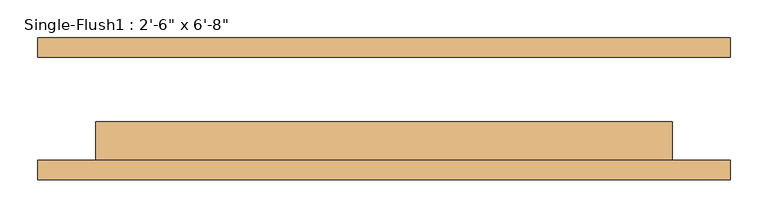
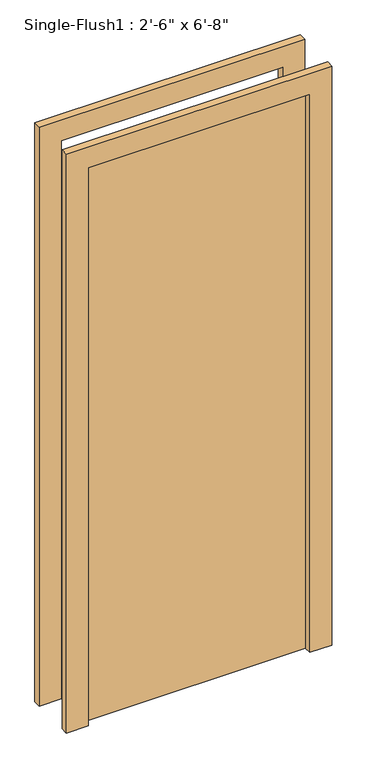
"""IFC4 building model written with IfcOpenShell, lengths in millimetres: door geometry."""

import ifcopenshell
import ifcopenshell.guid

model = None  # the IFC model being written
_history = None  # IfcOwnerHistory: only IFC2X3 demands one
_inside = {}  # id of a spatial element -> (the spatial element, [elements in it])
_under = {}  # id of a project, library or spatial element -> (it, [spatial elements below it])
_declared = {}  # id of a project -> (the project, [libraries it declares])
_typed = {}  # id of a type object -> (the type object, [elements of that type])
_made_of = {}  # id of a material, layer set ... -> (it, [elements and type objects made of it])


def new_model(schema):
    """Start an empty IFC model of exactly this schema.

    Asked for "IFC4X3", IfcOpenShell would pick the latest addendum, in which some entities
    have other attributes; the version numbers below select the first issue.
    IFC2X3 requires an IfcOwnerHistory on every rooted entity: one is made here for all.
    """
    global model, _history
    if schema == "IFC4X3":
        model = ifcopenshell.file(schema_version=(4, 3, 0, 0))
    else:
        model = ifcopenshell.file(schema=schema)
    _inside.clear()
    _under.clear()
    _declared.clear()
    _typed.clear()
    _made_of.clear()
    _history = None
    if model.schema == "IFC2X3":
        org = make("IfcOrganization", Name="unknown")
        user = make(
            "IfcPersonAndOrganization",
            ThePerson=make("IfcPerson", FamilyName="unknown"),
            TheOrganization=org,
        )
        app = make(
            "IfcApplication",
            ApplicationDeveloper=org,
            Version="unknown",
            ApplicationFullName="unknown",
            ApplicationIdentifier="unknown",
        )
        _history = make(
            "IfcOwnerHistory",
            OwningUser=user,
            OwningApplication=app,
            ChangeAction="ADDED",
            CreationDate=0,
        )
    return model


def make(cls, **values):
    """One entity of the class cls with the attributes given. An attribute that is None is left unset."""
    return model.create_entity(
        cls, **{name: value for name, value in values.items() if value is not None}
    )


def rooted(cls, **values):
    """An entity with a GlobalId (a new one), such as an element, a storey or a relation."""
    return make(cls, GlobalId=ifcopenshell.guid.new(), OwnerHistory=_history, **values)


def si_unit(unit_type, name, prefix=None):
    """IfcSIUnit, for example si_unit("LENGTHUNIT", "METRE", prefix="MILLI")."""
    return make("IfcSIUnit", UnitType=unit_type, Prefix=prefix, Name=name)


def assignment(units):
    """IfcUnitAssignment: the units of a project."""
    return None if units is None else make("IfcUnitAssignment", Units=units)


def point(xyz):
    """IfcCartesianPoint."""
    return None if xyz is None else make("IfcCartesianPoint", Coordinates=xyz)


def direction(xyz):
    """IfcDirection."""
    return None if xyz is None else make("IfcDirection", DirectionRatios=xyz)


def frame(location, z_axis=None, x_axis=None):
    """IfcAxis2Placement3D, a coordinate frame: its origin and axes. An axis left out is left unset."""
    return make(
        "IfcAxis2Placement3D",
        Location=point(location),
        Axis=direction(z_axis),
        RefDirection=direction(x_axis),
    )


def origin():
    """The frame at (0, 0, 0) with its axes left unset."""
    return frame((0.0, 0.0, 0.0))


def origin_with_axes():
    """The frame at (0, 0, 0) with the z axis (0, 0, 1) and the x axis (1, 0, 0) written out."""
    return frame((0.0, 0.0, 0.0), z_axis=(0.0, 0.0, 1.0), x_axis=(1.0, 0.0, 0.0))


def place(relative_to, where):
    """IfcLocalPlacement: puts the frame where relative to a parent placement (None: the world)."""
    return make(
        "IfcLocalPlacement", PlacementRelTo=relative_to, RelativePlacement=where
    )


def context(
    kind, dimensions, precision=None, world=None, true_north=None, identifier=None
):
    """IfcGeometricRepresentationContext, for example the 3D "Model" context."""
    return make(
        "IfcGeometricRepresentationContext",
        ContextIdentifier=identifier,
        ContextType=kind,
        CoordinateSpaceDimension=dimensions,
        Precision=precision,
        WorldCoordinateSystem=world,
        TrueNorth=true_north,
    )


def project(units=None, contexts=None):
    """IfcProject with its units and contexts."""
    return rooted(
        "IfcProject",
        Name="project",
        RepresentationContexts=contexts,
        UnitsInContext=assignment(units),
    )


def spatial(cls, under=None, at=None, **own):
    """A site, building, storey or space (cls), placed at a placement, below another one or the project."""
    s = rooted(cls, ObjectPlacement=at, **own)
    if under is not None:
        _under.setdefault(under.id(), (under, []))[1].append(s)
    return s


def polyline(points):
    """IfcPolyline through the points."""
    return make("IfcPolyline", Points=[point(p) for p in points])


def outline(outer, holes=None, kind="AREA"):
    """IfcArbitraryClosedProfileDef: a profile drawn as a closed curve; with holes, ...WithVoids."""
    if holes is None:
        return make("IfcArbitraryClosedProfileDef", ProfileType=kind, OuterCurve=outer)
    return make(
        "IfcArbitraryProfileDefWithVoids",
        ProfileType=kind,
        OuterCurve=outer,
        InnerCurves=holes,
    )


def extrude(swept, where, along, depth):
    """IfcExtrudedAreaSolid: the profile swept, set in the frame where, extruded along a direction by depth."""
    return make(
        "IfcExtrudedAreaSolid",
        SweptArea=swept,
        Position=where,
        ExtrudedDirection=direction(along),
        Depth=depth,
    )


def shape(context_of_items, identifier, shape_type, items):
    """IfcShapeRepresentation: the items that make up one representation, for example the "Body"."""
    return make(
        "IfcShapeRepresentation",
        ContextOfItems=context_of_items,
        RepresentationIdentifier=identifier,
        RepresentationType=shape_type,
        Items=items,
    )


def source(mapping_origin, context_of_items, identifier, shape_type, items):
    """IfcRepresentationMap: a shape defined once, which mapped items show again and again."""
    return make(
        "IfcRepresentationMap",
        MappingOrigin=mapping_origin,
        MappedRepresentation=shape(context_of_items, identifier, shape_type, items),
    )


def transform(
    local_origin,
    x_axis=None,
    y_axis=None,
    z_axis=None,
    scale=None,
    scale2=None,
    scale3=None,
    uniform=True,
):
    """IfcCartesianTransformationOperator3D, or its non-uniform kind. x_axis, y_axis, z_axis: its Axis1, 2, 3."""
    if uniform:
        return make(
            "IfcCartesianTransformationOperator3D",
            Axis1=direction(x_axis),
            Axis2=direction(y_axis),
            LocalOrigin=point(local_origin),
            Scale=scale,
            Axis3=direction(z_axis),
        )
    return make(
        "IfcCartesianTransformationOperator3DnonUniform",
        Axis1=direction(x_axis),
        Axis2=direction(y_axis),
        LocalOrigin=point(local_origin),
        Scale=scale,
        Axis3=direction(z_axis),
        Scale2=scale2,
        Scale3=scale3,
    )


def mapped(mapping_source, mapping_target):
    """IfcMappedItem: shows the shape of a source again, moved by a transform."""
    return make(
        "IfcMappedItem", MappingSource=mapping_source, MappingTarget=mapping_target
    )


def made_of(thing, what):
    """Note that an element or type object is made of a material, layer set ...; save() writes the relation."""
    if what is not None:
        _made_of.setdefault(what.id(), (what, []))[1].append(thing)
    return thing


def element(
    cls,
    number,
    at=None,
    inside=None,
    cuts=None,
    type_object=None,
    material=None,
    context=None,
    identifier="Body",
    shape_type=None,
    held_by="IfcProductDefinitionShape",
    body=None,
    shapes=None,
    **own,
):
    """One element of the class cls, such as IfcWall. Its Tag is "e" and its number.

    at: its placement. inside: the storey or other place that contains it. cuts: it is an
    opening in that element (IfcRelVoidsElement). A single representation is given by context,
    identifier, shape_type and body (its items); several are given by shapes. held_by: the class
    of the entity that holds the representations. save() writes the other relations.
    """
    e = rooted(cls, Tag="e%d" % number, ObjectPlacement=at, **own)
    if body is not None:
        shapes = [shape(context, identifier, shape_type, body)]
    if shapes is not None:
        e.Representation = make(held_by, Representations=shapes)
    if inside is not None:
        _inside.setdefault(inside.id(), (inside, []))[1].append(e)
    if cuts is not None:
        rooted(
            "IfcRelVoidsElement", RelatingBuildingElement=cuts, RelatedOpeningElement=e
        )
    if type_object is not None:
        _typed.setdefault(type_object.id(), (type_object, []))[1].append(e)
    return made_of(e, material)


def aggregate(whole, parts):
    """IfcRelAggregates: a whole, such as a stair, and the parts it consists of."""
    return rooted("IfcRelAggregates", RelatingObject=whole, RelatedObjects=parts)


def save(model, path):
    """Write the relations noted so far, then the file.

    IfcRelAggregates (storeys below a building ...), IfcRelContainedInSpatialStructure (elements
    in a storey), IfcRelDefinesByType, IfcRelAssociatesMaterial and IfcRelDeclares: one each for
    every whole, place, type object, material and project.
    """
    for whole, parts in _under.values():
        aggregate(whole, parts)
    for where, things in _inside.values():
        rooted(
            "IfcRelContainedInSpatialStructure",
            RelatedElements=things,
            RelatingStructure=where,
        )
    for kind, things in _typed.values():
        rooted("IfcRelDefinesByType", RelatedObjects=things, RelatingType=kind)
    for what, things in _made_of.values():
        rooted("IfcRelAssociatesMaterial", RelatedObjects=things, RelatingMaterial=what)
    for by, libraries in _declared.values():
        rooted("IfcRelDeclares", RelatingContext=by, RelatedDefinitions=libraries)
    model.write(path)


def door_cf295576(model_context):
    return source(origin(), model_context, "Body", "SweptSolid", [
        extrude(outline(polyline([(2108.2, -457.2), (0.0, -457.2), (0.0, -381.0), (2032.0, -381.0), (2032.0, 381.0), (0.0, 381.0), (0.0, 457.2), (2108.2, 457.2), (2108.2, -457.2)])), frame((0.0, -93.6625, 0.0), z_axis=(0.0, 1.0, 0.0), x_axis=(0.0, 0.0, 1.0)), (0.0, 0.0, 1.0), 25.4),
        extrude(outline(polyline([(2108.2, 457.2), (2108.2, -457.2), (0.0, -457.2), (0.0, -381.0), (2032.0, -381.0), (2032.0, 381.0), (0.0, 381.0), (0.0, 457.2), (2108.2, 457.2)])), frame((0.0, 68.2625, 0.0), z_axis=(0.0, 1.0, 0.0), x_axis=(0.0, 0.0, 1.0)), (0.0, 0.0, 1.0), 25.4),
        extrude(outline(polyline([(381.0, -17.4625), (381.0, -68.2625), (-381.0, -68.2625), (-381.0, -17.4625), (381.0, -17.4625)])), origin_with_axes(), (0.0, 0.0, 1.0), 2032.0),
    ])


if __name__ == "__main__":
    model = new_model("IFC4")
    model_context = context("Model", 3, world=origin())
    ifc_project = project(units=[si_unit("LENGTHUNIT", "METRE", prefix="MILLI")], contexts=[model_context])
    site = spatial("IfcSite", under=ifc_project)
    building = spatial("IfcBuilding", under=site)
    placement = place(None, origin())
    door_shape = door_cf295576(model_context)
    element("IfcDoor", 1, ObjectType="Single-Flush1 : 2'-6\" x 6'-8\"", at=placement, inside=building, context=model_context, shape_type="MappedRepresentation", body=[
        mapped(door_shape, transform((0.0, 0.0, 0.0), x_axis=(1.0, 0.0, 0.0), y_axis=(0.0, 1.0, 0.0), z_axis=(0.0, 0.0, 1.0))),
    ])
    save(model, "model.ifc")

# Revit data of these elements
# Type "Single-Flush1 : 2'-6\" x 6'-8\""
#   Type Mark = "D6"
#   Construction Type Id = "MDOOR"
#   Assembly Code = "C1020"
#   Analytic Construction = "Metal"
#   Thickness = 0' - 2"
#   Heat Transfer Coefficient (U) = 3.7021 W/(m²·K)
#   Height = 6' - 8"
#   Trim Projection Ext = 0' - 1"
#   Trim Projection Int = 0' - 1"
#   Trim Width = 0' - 3"
#   Width = 2' - 6"
#   Door Material = Door - Panel
#   Frame Material = Door - Frame
#   Visual Light Transmittance = 0
#   Solar Heat Gain Coefficient = 0
#   Function = (empty or 0)
#   Wall Closure = (empty or 0)
# Element 1 (IfcDoor, "Single-Flush1 : 2'-6\" x 6'-8\"")
#   Materials on its faces: "Door - Frame", "Door - Panel"
# Materials
#   "Door - Panel": class "Wood", colour RGB 210 159 95, transparency 0, Cost = 0
#   "Door - Frame": class "Miscellaneous", colour RGB 118 70 51, transparency 0, Cost = 0
